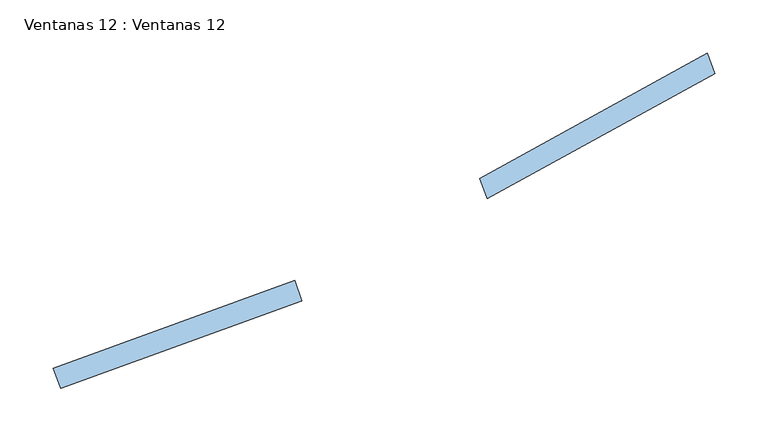
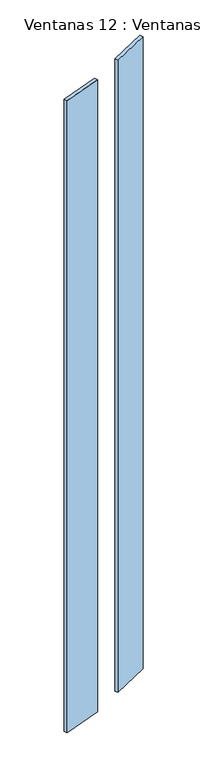
"""IFC4 building model written with IfcOpenShell, lengths in millimetres: window geometry, Ventanas 12 : Ventanas 12."""

from ifc_helpers import new_model, si_unit, frame, origin, place, context, project, spatial, polyline, outline, extrude, source, transform, mapped, element, save


def ventanas_12_ventanas_12_b765a59a(model_context):
    return source(origin(), model_context, "Body", "SweptSolid", [
        extrude(outline(polyline([(-5328.0123639, -5520.2868712), (-5321.1719611, -5539.0807236), (-5546.6981901, -5621.165558), (-5553.5385929, -5602.3717056), (-5328.0123639, -5520.2868712)])), frame((0.0, 0.0, 6223.3068472), z_axis=(0.0, 0.0, 1.0), x_axis=(1.0, 0.0, 0.0)), (0.0, 0.0, 1.0), 3883.9666763),
        extrude(outline(polyline([(-4942.1552109, -5307.5463382), (-4935.314808, -5326.3401907), (-5148.031014, -5443.6202739), (-5154.8714169, -5424.8264215), (-4942.1552109, -5307.5463382)])), frame((0.0, 0.0, 6223.3068472), z_axis=(0.0, 0.0, 1.0), x_axis=(1.0, 0.0, 0.0)), (0.0, 0.0, 1.0), 3883.9666763),
    ])


if __name__ == "__main__":
    model = new_model("IFC4")
    model_context = context("Model", 3, world=origin())
    ifc_project = project(units=[si_unit("LENGTHUNIT", "METRE", prefix="MILLI")], contexts=[model_context])
    site = spatial("IfcSite", under=ifc_project)
    building = spatial("IfcBuilding", under=site)
    placement = place(None, origin())
    ventanas_12_ventanas_12_shape = ventanas_12_ventanas_12_b765a59a(model_context)
    element("IfcWindow", 1, ObjectType="Ventanas 12 : Ventanas 12", at=placement, inside=building, context=model_context, shape_type="MappedRepresentation", body=[
        mapped(ventanas_12_ventanas_12_shape, transform((0.0, 0.0, 0.0), x_axis=(1.0, 0.0, 0.0), y_axis=(0.0, 1.0, 0.0), z_axis=(0.0, 0.0, 1.0))),
    ])
    save(model, "model.ifc")

# Revit data of these elements
# Type "Ventanas 12 : Ventanas 12"
#   Type Mark = "38"
# Element 1 (IfcWindow, "Ventanas 12 : Ventanas 12")
#   Materials on its faces: "VIDRIO"
# Materials
#   "VIDRIO": class "Genérico", colour RGB 120 120 120, transparency 0, Cost = 0
